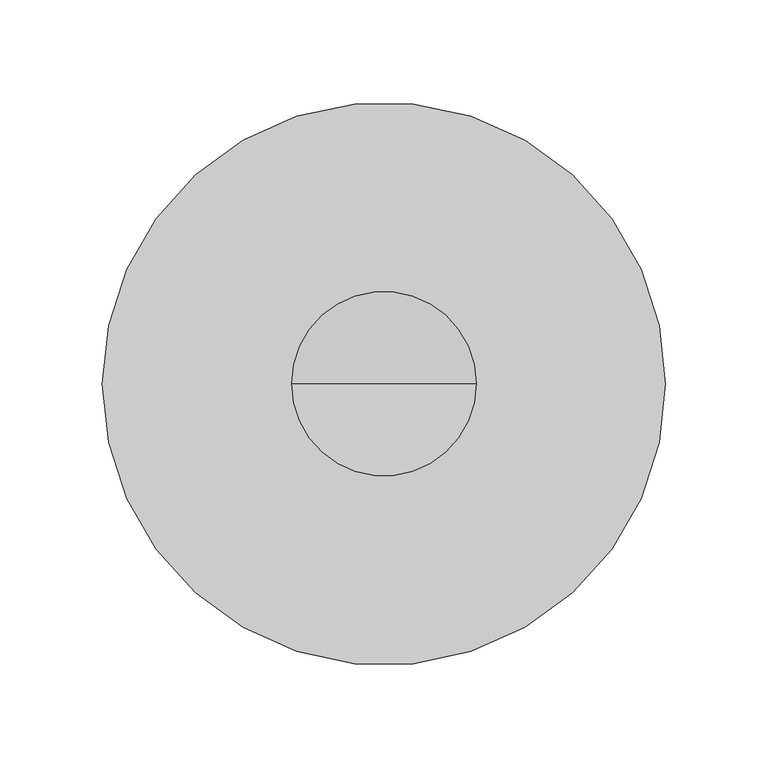
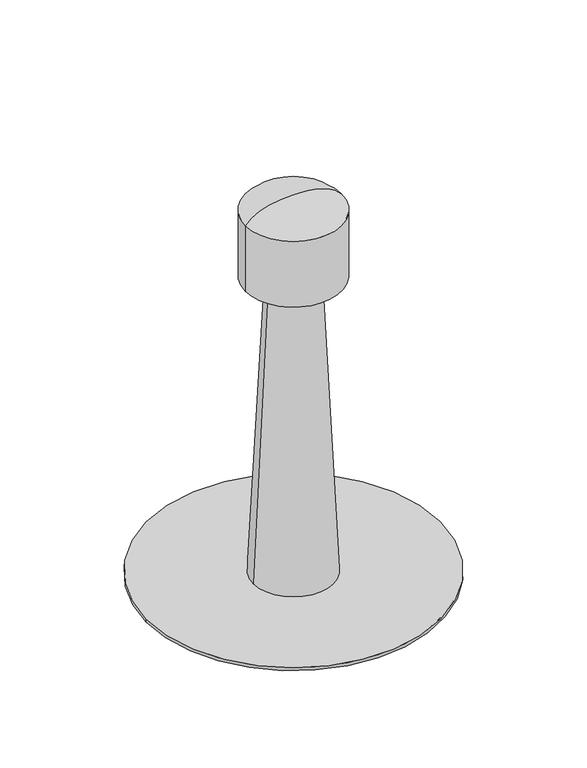
"""IFC4 building model written with IfcOpenShell, lengths in millimetres: proxy geometry, TN_ПВХ Кровельный аэратор : ПВХ аэратор кровельный Ultra 75х375 ТехноНИКОЛЬ."""

from ifc_helpers import new_model, si_unit, point, frame, origin, origin_with_axes, origin_2d, place, context, project, spatial, polyline, circle_curve, trimmed, segment, composite_curve, outline, extrude, source, transform, mapped, element, save
from ifc_brep_helpers import plane_surface, cylinder_surface, revolved_surface, spline_curve, advanced_brep


def specialty_equipment_3de617bf(model_context):
    return source(origin(), model_context, "Body", "SolidModel", [
        advanced_brep(
        [(23.5, 0.0, 295.0), (-23.5, 0.0, 295.0), (0.0, 0.0, 295.0), (0.0, 0.0, 3.0), (-37.5, 0.0, 3.0), (37.5, 0.0, 3.0)],
        [
            (0, 1, circle_curve(frame((0.0, 0.0, 295.0), z_axis=(0.0, 0.0, 1.0), x_axis=(-1.0, 0.0, 0.0)), 23.5)),
            (1, 2),
            (2, 0),
            (1, 0, circle_curve(frame((0.0, 0.0, 295.0), z_axis=(0.0, 0.0, 1.0), x_axis=(-1.0, 0.0, 0.0)), 23.5)),
            (3, 4),
            (4, 5, circle_curve(frame((0.0, 0.0, 3.0), z_axis=(0.0, 0.0, -1.0), x_axis=(-1.0, 0.0, 0.0)), 37.5)),
            (5, 3),
            (5, 4, circle_curve(frame((0.0, 0.0, 3.0), z_axis=(0.0, 0.0, -1.0), x_axis=(-1.0, 0.0, 0.0)), 37.5)),
            (4, 1),
            (0, 5),
        ],
        [
            plane_surface(frame((0.0, 0.0, 295.0), z_axis=(0.0, 0.0, 1.0), x_axis=(-1.0, 0.0, 0.0))),
            plane_surface(frame((0.0, 0.0, 3.0), z_axis=(0.0, 0.0, -1.0), x_axis=(-1.0, 0.0, 0.0))),
            revolved_surface(polyline([(-23.5, 0.0, 295.0), (-37.5, 0.0, 3.0)]), (0.0, 0.0, -2.0), (0.0, 0.0, -1.0)),
        ],
        [
            (0, [[1, 2, 3]]),
            (0, [[4, -3, -2]]),
            (1, [[5, 6, 7]]),
            (1, [[-7, 8, -5]]),
            (2, [[-6, 9, -1, 10]]),
            (2, [[-8, -10, -4, -9]]),
        ],
    ),
        advanced_brep(
        [(0.0, 0.0, 295.0), (-45.0, 0.0, 295.0), (45.0, 0.0, 295.0), (45.0, 0.0, 360.0), (-45.0, 0.0, 360.0), (0.0, 0.0, 375.0)],
        [
            (0, 1),
            (1, 2, circle_curve(frame((0.0, 0.0, 295.0), z_axis=(0.0, 0.0, -1.0), x_axis=(-1.0, 0.0, 0.0)), 45.0)),
            (2, 0),
            (2, 1, circle_curve(frame((0.0, 0.0, 295.0), z_axis=(0.0, 0.0, -1.0), x_axis=(-1.0, 0.0, 0.0)), 45.0)),
            (3, 4, circle_curve(frame((0.0, 0.0, 360.0), z_axis=(0.0, 0.0, 1.0), x_axis=(-1.0, 0.0, 0.0)), 45.0)),
            (4, 5, spline_curve(3, [(-45.0, 0.0, 360.0), (-36.982596383, 0.0, 369.999999999), (-21.982596382, 0.0, 375.0), (0.0, 0.0, 375.0)], [4, 4], [0.0, 0.08562924216502088])),
            (5, 3, spline_curve(3, [(0.0, 0.0, 375.0), (21.982596382, 0.0, 375.0), (36.982596383, 0.0, 369.999999999), (45.0, 0.0, 360.0)], [4, 4], [0.0, 0.08562924216502088])),
            (4, 3, circle_curve(frame((0.0, 0.0, 360.0), z_axis=(0.0, 0.0, 1.0), x_axis=(-1.0, 0.0, 0.0)), 45.0)),
            (1, 4),
            (3, 2),
        ],
        [
            plane_surface(frame((0.0, 0.0, 295.0), z_axis=(0.0, 0.0, -1.0), x_axis=(-1.0, 0.0, 0.0))),
            revolved_surface(spline_curve(3, [(0.0, 0.0, 375.0), (-21.982596382, 0.0, 375.0), (-36.982596383, 0.0, 369.999999999), (-45.0, 0.0, 360.0)], [4, 4], [0.0, 0.08562924216502088]), (0.0, 0.0, 390.0), (0.0, 0.0, -1.0)),
            cylinder_surface(frame((0.0, 0.0, 390.0), z_axis=(0.0, 0.0, -1.0), x_axis=(-1.0, 0.0, 0.0)), 45.0),
        ],
        [
            (0, [[1, 2, 3]]),
            (0, [[-3, 4, -1]]),
            (1, [[5, 6, 7]]),
            (1, [[8, -7, -6]]),
            (2, [[-2, 9, -5, 10]]),
            (2, [[-4, -10, -8, -9]]),
        ],
    ),
        extrude(outline(composite_curve([segment(trimmed(circle_curve(origin_2d(), 137.5), [point((-137.5, 0.0))], [point((137.5, 0.0))], False, "CARTESIAN"), True, "CONTINUOUS"), segment(trimmed(circle_curve(origin_2d(), 137.5), [point((137.5, 0.0))], [point((-137.5, 0.0))], False, "CARTESIAN"), True, "CONTINUOUS")], self_intersect=False)), origin_with_axes(), (0.0, 0.0, 1.0), 3.0),
    ])


if __name__ == "__main__":
    model = new_model("IFC4")
    model_context = context("Model", 3, world=origin())
    ifc_project = project(units=[si_unit("LENGTHUNIT", "METRE", prefix="MILLI")], contexts=[model_context])
    site = spatial("IfcSite", under=ifc_project)
    building = spatial("IfcBuilding", under=site)
    placement = place(None, origin())
    specialty_equipment_shape = specialty_equipment_3de617bf(model_context)
    element("IfcBuildingElementProxy", 1, Name="TN_ПВХ Кровельный аэратор : ПВХ аэратор кровельный Ultra 75х375 ТехноНИКОЛЬ", ObjectType="TN_ПВХ Кровельный аэратор : ПВХ аэратор кровельный Ultra 75х375 ТехноНИКОЛЬ", at=placement, inside=building, context=model_context, shape_type="MappedRepresentation", body=[
        mapped(specialty_equipment_shape, transform((0.0, 0.0, 0.0), x_axis=(1.0, 0.0, 0.0), y_axis=(0.0, 1.0, 0.0), z_axis=(0.0, 0.0, 1.0))),
    ])
    save(model, "model.ifc")

# Revit data of these elements
# Type "TN_ПВХ Кровельный аэратор : ПВХ аэратор кровельный Ultra 75х375 ТехноНИКОЛЬ"
#   Description = "ПВХ аэратор применяется при устройстве либо санации «дышащих» плоских кровель. Предназначены для отвода водяных паров, проникающих под гидроизоляционный слой кровли. Предотвращают образование вздутий и последующего разрыва защитного кровельного материала, тем самым увеличивая срок службы гидроизоляционного ковра.  Главным отличием от других существующих аэраторов является доработанная конструкция колпака, позволяющая выводить влагу быстрее.  Устанавливаются аэраторы данного типа из расчета не менее 1 шт. на 235 м² кровли. Расстояние между аэраторами не должно превышать 16,5 метров."
#   Manufacturer = "ТехноНИКОЛЬ"
#   URL = "https://shop.tn.ru/pvh-ajerator-krovelnyj-ultra-75h375-mm"
#   ADSK_Обозначение = "ТехноНИКОЛЬ"
#   ADSK_Наименование = "ПВХ аэратор кровельный Ultra 75х375мм"
#   ADSK_Код изделия = "55667"
#   ADSK_Завод-изготовитель = "ТехноНИКОЛЬ"
#   ADSK_Единица измерения = "шт."
#   ADSK_Группирование = "Комплектующие и воронки"
#   ADSK_URL страницы изделия = "https://shop.tn.ru/pvh-ajerator-krovelnyj-ultra-75h375-mm"
#   ADSK_URL документации изделия = "https://shop.tn.ru/pvh-ajerator-krovelnyj-ultra-75h375-mm"
#   Default Elevation = 1219.2 mm
#   ADSK_Размер_Ширина = 37.5 mm
#   ADSK_Размер_Высота = 375 mm
#   ADSK_Масса = 0.83
#   ADSK_Количество = 1
#   Материал = TN_ПВХ_ТемноСерый
# Element 1 (IfcBuildingElementProxy, "TN_ПВХ Кровельный аэратор : ПВХ аэратор кровельный Ultra 75х375 ТехноНИКОЛЬ")
#   Materials on its faces: "TN_ПВХ_ТемноСерый"
# Materials
#   "TN_ПВХ_ТемноСерый": class "Типовые", colour RGB 100 100 100, transparency 0, Cost = 0
